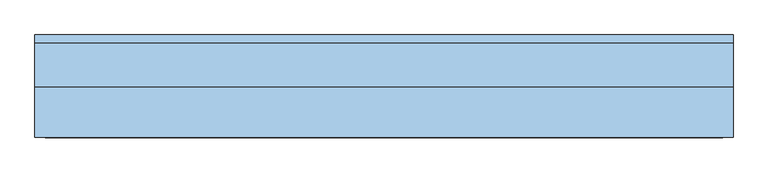
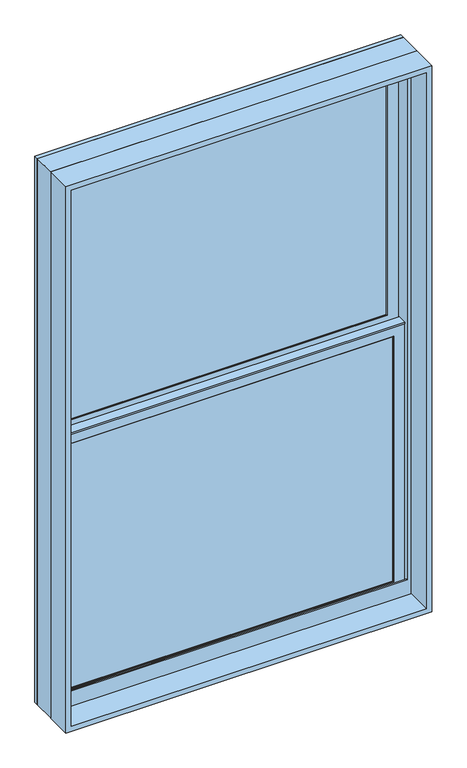
"""IFC4 building model written with IfcOpenShell, lengths in millimetres: window geometry, Window-Double_Hung-Marvin-Essential : ESDH3656."""

from ifc_helpers import new_model, si_unit, frame, origin, place, context, project, spatial, polyline, outline, extrude, faceted_brep, source, transform, mapped, element, save


def window_9ba8db7a(model_context):
    return source(origin(), model_context, "Body", "SolidModel", [
        extrude(outline(polyline([(166.1583333, 20.6375), (166.1583333, 15.875), (147.1083333, 15.875), (147.1083333, 20.6375), (166.1583333, 20.6375)])), frame((0.0, 0.0, 831.85), z_axis=(0.0, 0.0, 1.0), x_axis=(1.0, 0.0, 0.0)), (0.0, 0.0, 1.0), 755.65),
        extrude(outline(polyline([(-147.1083333, 20.6375), (-147.1083333, 15.875), (-166.1583333, 15.875), (-166.1583333, 20.6375), (-147.1083333, 20.6375)])), frame((0.0, 0.0, 831.85), z_axis=(0.0, 0.0, 1.0), x_axis=(1.0, 0.0, 0.0)), (0.0, 0.0, 1.0), 755.65),
        extrude(outline(polyline([(469.9, 20.6375), (469.9, 15.875), (-469.9, 15.875), (-469.9, 20.6375), (469.9, 20.6375)])), frame((0.0, 0.0, 1200.15), z_axis=(0.0, 0.0, 1.0), x_axis=(1.0, 0.0, 0.0)), (0.0, 0.0, 1.0), 19.05),
        extrude(outline(polyline([(-166.1583333, 46.83125), (-166.1583333, 51.59375), (-147.1083333, 51.59375), (-147.1083333, 46.83125), (-166.1583333, 46.83125)])), frame((0.0, 0.0, 1625.6), z_axis=(0.0, 0.0, 1.0), x_axis=(1.0, 0.0, 0.0)), (0.0, 0.0, 1.0), 755.65),
        extrude(outline(polyline([(147.1083333, 46.83125), (147.1083333, 51.59375), (166.1583333, 51.59375), (166.1583333, 46.83125), (147.1083333, 46.83125)])), frame((0.0, 0.0, 1625.6), z_axis=(0.0, 0.0, 1.0), x_axis=(1.0, 0.0, 0.0)), (0.0, 0.0, 1.0), 755.65),
        extrude(outline(polyline([(-469.9, 46.83125), (-469.9, 51.59375), (469.9, 51.59375), (469.9, 46.83125), (-469.9, 46.83125)])), frame((0.0, 0.0, 1993.9), z_axis=(0.0, 0.0, 1.0), x_axis=(1.0, 0.0, 0.0)), (0.0, 0.0, 1.0), 19.05),
        extrude(outline(polyline([(166.1583333, 20.6375), (147.1083333, 20.6375), (147.1083333, 25.4), (166.1583333, 25.4), (166.1583333, 20.6375)])), frame((0.0, 0.0, 831.85), z_axis=(0.0, 0.0, 1.0), x_axis=(1.0, 0.0, 0.0)), (0.0, 0.0, 1.0), 755.65),
        extrude(outline(polyline([(-147.1083333, 20.6375), (-166.1583333, 20.6375), (-166.1583333, 25.4), (-147.1083333, 25.4), (-147.1083333, 20.6375)])), frame((0.0, 0.0, 831.85), z_axis=(0.0, 0.0, 1.0), x_axis=(1.0, 0.0, 0.0)), (0.0, 0.0, 1.0), 755.65),
        extrude(outline(polyline([(469.9, 20.6375), (-469.9, 20.6375), (-469.9, 25.4), (469.9, 25.4), (469.9, 20.6375)])), frame((0.0, 0.0, 1200.15), z_axis=(0.0, 0.0, 1.0), x_axis=(1.0, 0.0, 0.0)), (0.0, 0.0, 1.0), 19.05),
        extrude(outline(polyline([(-166.1583333, 56.35625), (-147.1083333, 56.35625), (-147.1083333, 51.59375), (-166.1583333, 51.59375), (-166.1583333, 56.35625)])), frame((0.0, 0.0, 1625.6), z_axis=(0.0, 0.0, 1.0), x_axis=(1.0, 0.0, 0.0)), (0.0, 0.0, 1.0), 755.65),
        extrude(outline(polyline([(147.1083333, 56.35625), (166.1583333, 56.35625), (166.1583333, 51.59375), (147.1083333, 51.59375), (147.1083333, 56.35625)])), frame((0.0, 0.0, 1625.6), z_axis=(0.0, 0.0, 1.0), x_axis=(1.0, 0.0, 0.0)), (0.0, 0.0, 1.0), 755.65),
        extrude(outline(polyline([(-469.9, 56.35625), (469.9, 56.35625), (469.9, 51.59375), (-469.9, 51.59375), (-469.9, 56.35625)])), frame((0.0, 0.0, 1993.9), z_axis=(0.0, 0.0, 1.0), x_axis=(1.0, 0.0, 0.0)), (0.0, 0.0, 1.0), 19.05),
        faceted_brep([(-496.8875, 5.6780605, 1617.5351748), (-496.8875, 5.6780605, 1612.9), (496.8875, 5.6780605, 1612.9), (496.8875, 5.6780605, 1617.5351748), (-496.8875, 34.8118605, 1617.5351748), (496.8875, 34.8118605, 1617.5351748), (496.8875, 34.8118605, 1612.9), (-496.8875, 34.8118605, 1612.9), (-496.8875, 30.1625, 1612.9), (-496.8875, 30.1625, 804.8625), (-496.8875, 8.9241104, 804.8625), (-496.8875, 8.9241104, 1612.9), (496.8875, 8.9241104, 1612.9), (496.8875, 30.1625, 1612.9), (496.8875, 8.9241104, 804.8625), (496.8875, 30.1625, 804.8625), (-481.0034752, 11.90625, 1598.6034752), (-481.0034752, 30.1625, 1598.6034752), (481.0034752, 30.1625, 1598.6034752), (481.0034752, 11.90625, 1598.6034752), (-464.34375, 10.4662439, 1581.94375), (-464.34375, 11.90625, 1581.94375), (464.34375, 11.90625, 1581.94375), (464.34375, 10.4662439, 1581.94375), (465.8858834, 8.9241104, 1583.4858834), (-465.8858834, 8.9241104, 1583.4858834), (481.0034752, 30.1625, 820.7465248), (481.0034752, 11.90625, 820.7465248), (464.34375, 11.90625, 837.40625), (464.34375, 10.4662439, 837.40625), (465.8858834, 8.9241104, 835.8641166), (-481.0034752, 30.1625, 820.7465248), (-481.0034752, 11.90625, 820.7465248), (-464.34375, 11.90625, 837.40625), (-464.34375, 10.4662439, 837.40625), (-465.8858834, 8.9241104, 835.8641166)], [[[0, 1, 2, 3]], [[4, 5, 6, 7]], [[1, 0, 4, 7, 8, 9, 10, 11]], [[2, 1, 11, 12]], [[7, 6, 13, 8]], [[3, 2, 12, 14, 15, 13, 6, 5]], [[0, 3, 5, 4]], [[16, 17, 18, 19]], [[20, 21, 22, 23]], [[20, 23, 24, 25]], [[19, 18, 26, 27]], [[23, 22, 28, 29]], [[24, 23, 29, 30]], [[27, 26, 31, 32]], [[29, 28, 33, 34]], [[30, 29, 34, 35]], [[15, 14, 10, 9]], [[15, 9, 8, 13], [18, 17, 31, 26]], [[17, 16, 32, 31]], [[16, 19, 27, 32], [22, 21, 33, 28]], [[21, 20, 34, 33]], [[20, 25, 35, 34]], [[10, 14, 12, 11], [25, 24, 30, 35]]]),
        extrude(outline(polyline([(38.5955581, 1598.6125), (33.5778968, 1598.6125), (33.5778968, 1600.2), (39.9405976, 1600.2), (39.9405976, 1598.6125), (61.515625, 1598.6125), (47.6307501, 1595.2975159), (38.5955581, 1595.2975159), (38.5955581, 1598.6125)])), frame((-496.8875, 0.0, 0.0), z_axis=(1.0, 0.0, 0.0), x_axis=(0.0, 1.0, 0.0)), (0.0, 0.0, 1.0), 993.775),
        faceted_brep([(527.05, 0.0, 774.7), (527.05, 0.0, 2438.4), (-527.05, 0.0, 2438.4), (-527.05, 0.0, 774.7), (500.85625, 0.0, 835.81875), (-500.85625, 0.0, 835.81875), (-500.85625, 0.0, 2412.20625), (500.85625, 0.0, 2412.20625), (500.85625, 3.96875, 774.7), (-500.85625, 3.96875, 774.7), (-500.85625, 3.96875, 835.81875), (500.85625, 3.96875, 835.81875), (-527.05, 65.6828125, 774.7), (-500.85625, 65.6828125, 774.7), (500.85625, 65.6828125, 774.7), (527.05, 65.6828125, 774.7), (-527.05, 65.6828125, 2438.4), (527.05, 65.6828125, 2438.4), (500.85625, 65.6828125, 2412.20625), (-500.85625, 65.6828125, 2412.20625)], [[[0, 1, 2, 3], [4, 5, 6, 7]], [[8, 9, 10, 11]], [[5, 4, 11, 10]], [[0, 3, 12, 13, 9, 8, 14, 15]], [[13, 12, 16, 17, 15, 14, 18, 19]], [[13, 19, 6, 5, 10, 9]], [[7, 6, 19, 18]], [[18, 14, 8, 11, 4, 7]], [[1, 0, 15, 17]], [[2, 1, 17, 16]], [[3, 2, 16, 12]]]),
        faceted_brep([(500.85625, 30.1625, 1606.55), (499.26875, 30.1625, 1606.55), (499.26875, 30.1625, 799.0544613), (500.85625, 30.1625, 799.0544613), (-499.26875, 30.1625, 1606.55), (-500.85625, 30.1625, 1606.55), (-500.85625, 30.1625, 799.0544613), (-499.26875, 30.1625, 799.0544613), (499.26875, 63.5, 1606.55), (500.85625, 63.5, 1606.55), (500.85625, 63.5, 792.5743077), (499.26875, 63.5, 792.5743077), (-500.85625, 63.5, 1606.55), (-499.26875, 63.5, 1606.55), (-499.26875, 63.5, 792.5743077), (-500.85625, 63.5, 792.5743077), (512.1108932, 3.96875, 804.1460105), (512.1108932, 3.96875, 774.7), (512.1108932, 65.6828125, 774.7), (512.1108932, 65.6828125, 792.150012), (-512.1108932, 3.96875, 774.7), (-512.1108932, 3.96875, 804.1460105), (-512.1108932, 65.6828125, 792.150012), (-512.1108932, 65.6828125, 774.7), (512.1108932, 78.58125, 789.6428097), (-512.1108932, 78.58125, 789.6428097), (-510.0971252, 68.2348864, 791.6539391), (-492.13135, 68.2348864, 791.6539391), (-492.13135, 65.6828125, 792.150012), (492.13135, 65.6828125, 792.150012), (492.13135, 68.2348864, 791.6539391), (510.0971252, 68.2348864, 791.6539391), (-527.05, 65.6828125, 774.7), (-527.05, 78.5948249, 774.7), (527.05, 78.5948249, 774.7), (527.05, 65.6828125, 774.7), (-527.05, 78.58125, 2438.4), (527.05, 78.58125, 2438.4), (512.1108932, 78.58125, 2423.4608932), (-512.1108932, 78.58125, 2423.4608932), (-527.05, 65.6828125, 2438.4), (-510.0971252, 68.2348864, 2421.4471252), (510.0971252, 68.2348864, 2421.4471252), (492.13135, 68.2348864, 2403.48135), (-492.13135, 68.2348864, 2403.48135), (-492.13135, 65.6828125, 2403.48135), (492.13135, 65.6828125, 2403.48135), (527.05, 65.6828125, 2438.4)], [[[0, 1, 2, 3]], [[4, 5, 6, 7]], [[8, 9, 10, 11]], [[12, 13, 14, 15]], [[1, 8, 11, 2]], [[9, 0, 3, 10]], [[1, 0, 9, 8]], [[5, 4, 13, 12]], [[5, 12, 15, 6]], [[13, 4, 7, 14]], [[16, 17, 18, 19]], [[20, 21, 22, 23]], [[24, 25, 26, 27, 28, 22, 21, 16, 19, 29, 30, 31], [3, 2, 11, 10], [7, 6, 15, 14]], [[17, 16, 21, 20]], [[17, 20, 23, 32, 33, 34, 35, 18]], [[34, 33, 36, 37], [25, 24, 38, 39]], [[33, 32, 40, 36]], [[39, 41, 26, 25]], [[41, 42, 31, 30, 43, 44, 27, 26]], [[44, 45, 28, 27]], [[40, 32, 23, 22, 28, 45, 46, 29, 19, 18, 35, 47]], [[36, 40, 47, 37]], [[39, 38, 42, 41]], [[44, 43, 46, 45]], [[34, 37, 47, 35]], [[42, 38, 24, 31]], [[46, 43, 30, 29]]]),
        extrude(outline(polyline([(477.04375, 11.90625), (-477.04375, 11.90625), (-477.04375, 15.08125), (477.04375, 15.08125), (477.04375, 11.90625)])), frame((0.0, 0.0, 824.70625), z_axis=(0.0, 0.0, 1.0), x_axis=(1.0, 0.0, 0.0)), (0.0, 0.0, 1.0), 769.9375),
        extrude(outline(polyline([(477.04375, 42.8625), (-477.04375, 42.8625), (-477.04375, 46.0375), (477.04375, 46.0375), (477.04375, 42.8625)])), frame((0.0, 0.0, 1618.45625), z_axis=(0.0, 0.0, 1.0), x_axis=(1.0, 0.0, 0.0)), (0.0, 0.0, 1.0), 769.9375),
        faceted_brep([(-464.34375, 31.194477, 1581.94375), (-465.8858834, 32.7366104, 1583.4858834), (465.8858834, 32.7366104, 1583.4858834), (464.34375, 31.194477, 1581.94375), (-464.34375, 30.1625, 1581.94375), (464.34375, 30.1625, 1581.94375), (-496.8875, 32.7366104, 1614.4875), (-496.8875, 30.1625, 1614.4875), (496.8875, 30.1625, 1614.4875), (496.8875, 32.7366104, 1614.4875), (465.8858834, 32.7366104, 835.8641166), (464.34375, 31.194477, 837.40625), (464.34375, 30.1625, 837.40625), (496.8875, 30.1625, 804.8625), (496.8875, 32.7366104, 804.8625), (-465.8858834, 32.7366104, 835.8641166), (-464.34375, 31.194477, 837.40625), (-464.34375, 30.1625, 837.40625), (-496.8875, 30.1625, 804.8625), (-496.8875, 32.7366104, 804.8625)], [[[0, 1, 2, 3]], [[4, 0, 3, 5]], [[6, 7, 8, 9]], [[3, 2, 10, 11]], [[5, 3, 11, 12]], [[9, 8, 13, 14]], [[11, 10, 15, 16]], [[12, 11, 16, 17]], [[14, 13, 18, 19]], [[9, 14, 19, 6], [1, 15, 10, 2]], [[16, 15, 1, 0]], [[17, 16, 0, 4]], [[7, 18, 13, 8], [5, 12, 17, 4]], [[19, 18, 7, 6]]]),
        faceted_brep([(-481.0034752, 42.8625, 2392.3534752), (-481.0034752, 61.11875, 2392.3534752), (481.0034752, 61.11875, 2392.3534752), (481.0034752, 42.8625, 2392.3534752), (-464.34375, 41.4224939, 2375.69375), (-464.34375, 42.8625, 2375.69375), (464.34375, 42.8625, 2375.69375), (464.34375, 41.4224939, 2375.69375), (-465.8858834, 39.8803604, 2377.2358834), (465.8858834, 39.8803604, 2377.2358834), (-496.8875, 61.11875, 2408.2375), (-496.8875, 39.8803604, 2408.2375), (496.8875, 39.8803604, 2408.2375), (496.8875, 61.11875, 2408.2375), (481.0034752, 61.11875, 1614.4965248), (481.0034752, 42.8625, 1614.4965248), (464.34375, 42.8625, 1631.15625), (464.34375, 41.4224939, 1631.15625), (465.8858834, 39.8803604, 1629.6141166), (496.8875, 39.8803604, 1598.6125), (496.8875, 61.11875, 1598.6125), (-481.0034752, 61.11875, 1614.4965248), (-481.0034752, 42.8625, 1614.4965248), (-464.34375, 42.8625, 1631.15625), (-464.34375, 41.4224939, 1631.15625), (-465.8858834, 39.8803604, 1629.6141166), (-496.8875, 39.8803604, 1598.6125), (-496.8875, 61.11875, 1598.6125)], [[[0, 1, 2, 3]], [[4, 5, 6, 7]], [[8, 4, 7, 9]], [[10, 11, 12, 13]], [[3, 2, 14, 15]], [[7, 6, 16, 17]], [[9, 7, 17, 18]], [[13, 12, 19, 20]], [[15, 14, 21, 22]], [[17, 16, 23, 24]], [[18, 17, 24, 25]], [[20, 19, 26, 27]], [[13, 20, 27, 10], [1, 21, 14, 2]], [[22, 21, 1, 0]], [[3, 15, 22, 0], [5, 23, 16, 6]], [[24, 23, 5, 4]], [[25, 24, 4, 8]], [[11, 26, 19, 12], [9, 18, 25, 8]], [[27, 26, 11, 10]]]),
        faceted_brep([(-496.8875, 61.11875, 1598.6125), (-496.8875, 63.6928604, 1598.6125), (496.8875, 63.6928604, 1598.6125), (496.8875, 61.11875, 1598.6125), (-464.34375, 62.150727, 1631.15625), (-464.34375, 61.11875, 1631.15625), (464.34375, 61.11875, 1631.15625), (464.34375, 62.150727, 1631.15625), (-465.8858834, 63.6928604, 1629.6141166), (465.8858834, 63.6928604, 1629.6141166), (496.8875, 63.6928604, 2408.2375), (496.8875, 61.11875, 2408.2375), (464.34375, 61.11875, 2375.69375), (464.34375, 62.150727, 2375.69375), (465.8858834, 63.6928604, 2377.2358834), (-496.8875, 63.6928604, 2408.2375), (-496.8875, 61.11875, 2408.2375), (-464.34375, 61.11875, 2375.69375), (-464.34375, 62.150727, 2375.69375), (-465.8858834, 63.6928604, 2377.2358834)], [[[0, 1, 2, 3]], [[4, 5, 6, 7]], [[8, 4, 7, 9]], [[3, 2, 10, 11]], [[7, 6, 12, 13]], [[9, 7, 13, 14]], [[11, 10, 15, 16]], [[13, 12, 17, 18]], [[14, 13, 18, 19]], [[16, 15, 1, 0]], [[3, 11, 16, 0], [5, 17, 12, 6]], [[18, 17, 5, 4]], [[19, 18, 4, 8]], [[1, 15, 10, 2], [9, 14, 19, 8]]]),
        extrude(outline(polyline([(477.04375, 26.19375), (-477.04375, 26.19375), (-477.04375, 30.1625), (477.04375, 30.1625), (477.04375, 26.19375)])), frame((0.0, 0.0, 824.70625), z_axis=(0.0, 0.0, 1.0), x_axis=(1.0, 0.0, 0.0)), (0.0, 0.0, 1.0), 769.9375),
        extrude(outline(polyline([(477.04375, 57.15), (-477.04375, 57.15), (-477.04375, 61.11875), (477.04375, 61.11875), (477.04375, 57.15)])), frame((0.0, 0.0, 1618.45625), z_axis=(0.0, 0.0, 1.0), x_axis=(1.0, 0.0, 0.0)), (0.0, 0.0, 1.0), 769.9375),
        extrude(outline(polyline([(2438.4, 527.05), (2438.4, -527.05), (774.7, -527.05), (774.7, 527.05), (2438.4, 527.05)]), holes=[polyline([(2422.525, 511.175), (790.575, 511.175), (790.575, -511.175), (2422.525, -511.175), (2422.525, 511.175)])]), frame((0.0, -76.2, 0.0), z_axis=(0.0, 1.0, 0.0), x_axis=(0.0, 0.0, 1.0)), (0.0, 0.0, 1.0), 75.40625),
    ])


if __name__ == "__main__":
    model = new_model("IFC4")
    model_context = context("Model", 3, world=origin())
    ifc_project = project(units=[si_unit("LENGTHUNIT", "METRE", prefix="MILLI")], contexts=[model_context])
    site = spatial("IfcSite", under=ifc_project)
    building = spatial("IfcBuilding", under=site)
    placement = place(None, origin())
    window_shape = window_9ba8db7a(model_context)
    element("IfcWindow", 1, ObjectType="Window-Double_Hung-Marvin-Essential : ESDH3656", at=placement, inside=building, context=model_context, shape_type="MappedRepresentation", body=[
        mapped(window_shape, transform((0.0, 0.0, 0.0), x_axis=(1.0, 0.0, 0.0), y_axis=(0.0, 1.0, 0.0), z_axis=(0.0, 0.0, 1.0))),
    ])
    save(model, "model.ifc")

# Revit data of these elements
# Type "Window-Double_Hung-Marvin-Essential : ESDH3656"
#   Type Mark = "73"
#   Window Type = "Essential Double Hung"
#   Product data url = "https://bimobject.com/marvin-windows-and-doors/product/marvin-dhwau"
#   Product Guid = "c4a96547-874c-4385-91dc-a058adc19d98"
#   Frame = "All Ultrex"
#   Egress Window = "Yes"
#   URL = "www.marvin.com"
#   Model = "ESDH3656"
#   Manufacturer = "Marvin Windows and Doors"
#   Label Egress = "EGRESS WDW"
#   Glass Type = "IG Low E II with Argon"
#   Design Pressure = "DP40"
#   Description = "4266 DBHG"
#   Analytic Construction = "<None>"
#   Prairie Corner Width = 0' - 4"
#   Prairie Corner Height = 0' - 4"
#   Egress Width = 3' - 2 9/16"
#   Egress Height = 2' - 4 27/128"
#   Rough Width = 3' - 6"
#   Rough Height = 5' - 6"
#   Nominal Width = 3' - 6"
#   Nominal Height = 5' - 6"
#   Inset to Installation Flange [instance default] = 0' - 1"
#   Height = 5' - 5 1/2"
#   Egress Area = 7.55475 SF
#   Default Head Height = 8' - 0"
#   Width = 3' - 5 1/2"
#   Daylight Area = 14.8853 SF
#   DLO Width = 3' - 0 9/16"
#   DLO Height = 2' - 5 5/16"
#   Muntins Top Sash = yes
#   Lites Wide Top Sash = 3
#   Lites Wide Bottom Sash = 3
#   Lites High Top Sash = 2
#   Lites High Bottom Sash = 2
#   Lite Cut Prairie 9 = no
#   Lite Cut HV Grid = yes
#   Muntins Bottom Sash = yes
#   Label Visibility = no
#   Jamb Extension Visibility = yes
#   Edition number = 1
#   Interior Material = Ultrex-Marvin-Stonewhite
#   Glazing Material = Glass-Marvin-IG Low E II with Argon
#   Cladding Material = Ultrex-Marvin-Pebblegray
#   Wall Closure = (empty or 0)
#   Assembly Code = ""
# Element 1 (IfcWindow, "Window-Double_Hung-Marvin-Essential : ESDH3656")
#   Materials on its faces: "Ultrex-Marvin-Pebblegray", "Ultrex-Marvin-Stonewhite", "Glass-Marvin-IG Low E II with Argon"
# Materials
#   "Ultrex-Marvin-Stonewhite": class "Paint", colour RGB 250 251 245, transparency 0
#   "Glass-Marvin-IG Low E II with Argon": class "Glass", colour RGB 0 128 192, transparency 0.85
#   "Ultrex-Marvin-Pebblegray": class "Paint", colour RGB 189 185 173, transparency 0
